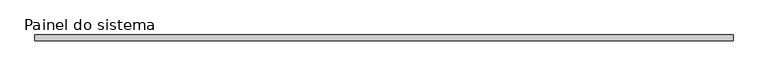
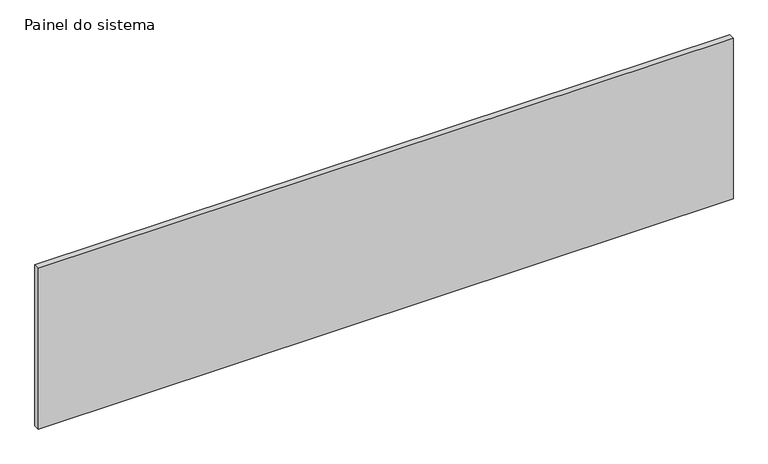
"""IFC4 building model written with IfcOpenShell, lengths in millimetres: plate geometry, Painel do sistema : Envidraçado."""

from ifc_helpers import new_model, si_unit, origin, origin_with_axes, place, context, project, spatial, polyline, outline, extrude, source, transform, mapped, element, save


def painel_do_sistema_cd1f443e(model_context):
    return source(origin(), model_context, "Body", "SweptSolid", [
        extrude(outline(polyline([(1487.5000075, 24.5), (-1487.5000075, 24.5), (-1487.5000075, 49.5), (1487.5000075, 49.5), (1487.5000075, 24.5)])), origin_with_axes(), (0.0, 0.0, 1.0), 727.4383788),
    ])


if __name__ == "__main__":
    model = new_model("IFC4")
    model_context = context("Model", 3, world=origin())
    ifc_project = project(units=[si_unit("LENGTHUNIT", "METRE", prefix="MILLI")], contexts=[model_context])
    site = spatial("IfcSite", under=ifc_project)
    building = spatial("IfcBuilding", under=site)
    placement = place(None, origin())
    painel_do_sistema_shape = painel_do_sistema_cd1f443e(model_context)
    element("IfcPlate", 1, ObjectType="Painel do sistema : Envidraçado", at=placement, inside=building, context=model_context, shape_type="MappedRepresentation", body=[
        mapped(painel_do_sistema_shape, transform((0.0, 0.0, 0.0), x_axis=(1.0, 0.0, 0.0), y_axis=(0.0, 1.0, 0.0), z_axis=(0.0, 0.0, 1.0))),
    ])
    save(model, "model.ifc")

# Revit data of these elements
# Type "Painel do sistema : Envidraçado"
#   Construction Type Id = "GSP4R"
#   Analytic Construction = "Vidraça única Pilkington 1/8 pol"
#   Visual Light Transmittance = 0.9
#   Solar Heat Gain Coefficient = 0.86
#   Heat Transfer Coefficient (U) = 6.7069 W/(m²·K)
# Element 1 (IfcPlate, "Painel do sistema : Envidraçado")
#   Materials on its faces: "Vidro"
# Materials
#   "Vidro": class "Vidro", colour RGB 0 128 192, transparency 0.9, Description = "Vidro de sílica", Cost = 0
